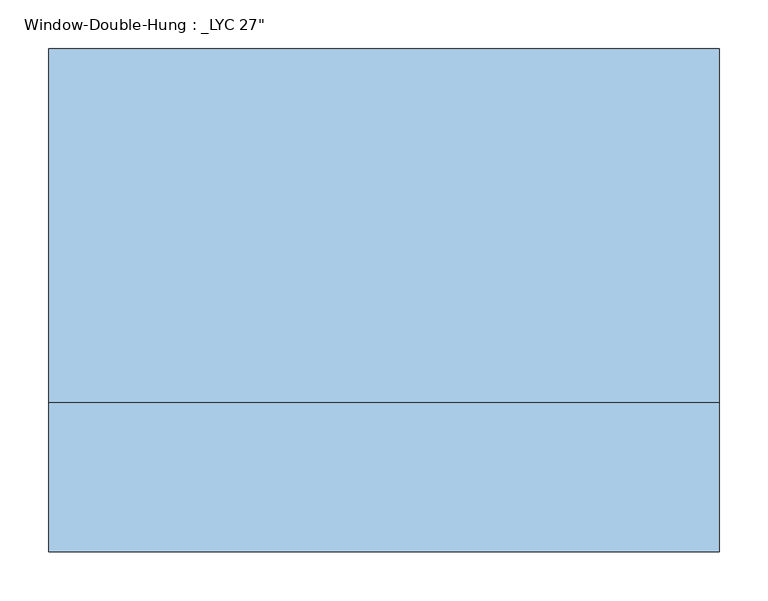
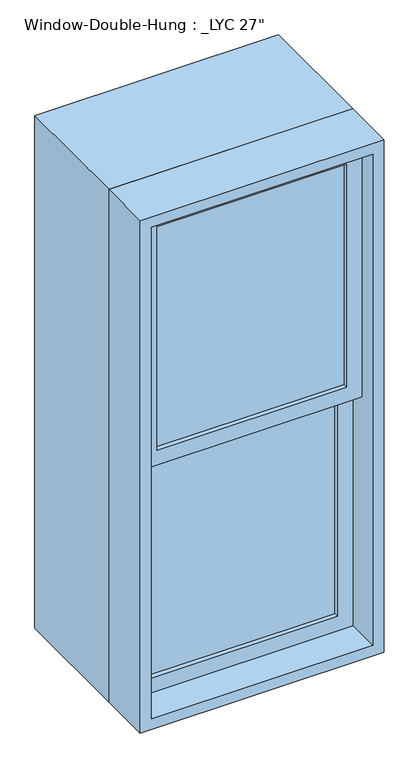
"""IFC4 building model written with IfcOpenShell, lengths in millimetres: window geometry."""

from ifc_helpers import new_model, si_unit, frame, origin, place, context, project, spatial, polyline, outline, extrude, source, transform, mapped, element, save


def window_2f9f7d73(model_context):
    return source(origin(), model_context, "Body", "SweptSolid", [
        extrude(outline(polyline([(266.7, -158.75), (-266.7, -158.75), (-266.7, -152.4), (266.7, -152.4), (266.7, -158.75)])), frame((0.0, 0.0, 990.6), z_axis=(0.0, 0.0, 1.0), x_axis=(1.0, 0.0, 0.0)), (0.0, 0.0, 1.0), 663.575),
        extrude(outline(polyline([(-266.7, -146.05), (-266.7, -139.7), (266.7, -139.7), (266.7, -146.05), (-266.7, -146.05)])), frame((0.0, 0.0, 990.6), z_axis=(0.0, 0.0, 1.0), x_axis=(1.0, 0.0, 0.0)), (0.0, 0.0, 1.0), 663.575),
        extrude(outline(polyline([(266.7, -203.2), (-266.7, -203.2), (-266.7, -196.85), (266.7, -196.85), (266.7, -203.2)])), frame((0.0, 0.0, 1698.625), z_axis=(0.0, 0.0, 1.0), x_axis=(1.0, 0.0, 0.0)), (0.0, 0.0, 1.0), 663.575),
        extrude(outline(polyline([(-266.7, -190.5), (-266.7, -184.15), (266.7, -184.15), (266.7, -190.5), (-266.7, -190.5)])), frame((0.0, 0.0, 1698.625), z_axis=(0.0, 0.0, 1.0), x_axis=(1.0, 0.0, 0.0)), (0.0, 0.0, 1.0), 663.575),
        extrude(outline(polyline([(1698.625, 311.15), (1698.625, -311.15), (946.15, -311.15), (946.15, 311.15), (1698.625, 311.15)]), holes=[polyline([(1654.175, -266.7), (1654.175, 266.7), (990.6, 266.7), (990.6, -266.7), (1654.175, -266.7)])]), frame((0.0, -171.45, 0.0), z_axis=(0.0, 1.0, 0.0), x_axis=(0.0, 0.0, 1.0)), (0.0, 0.0, 1.0), 44.45),
        extrude(outline(polyline([(2406.65, 311.15), (2406.65, -311.15), (1654.175, -311.15), (1654.175, 311.15), (2406.65, 311.15)]), holes=[polyline([(2362.2, -266.7), (2362.2, 266.7), (1698.625, 266.7), (1698.625, -266.7), (2362.2, -266.7)])]), frame((0.0, -215.9, 0.0), z_axis=(0.0, 1.0, 0.0), x_axis=(0.0, 0.0, 1.0)), (0.0, 0.0, 1.0), 44.45),
        extrude(outline(polyline([(2438.4, 342.9), (2438.4, -342.9), (914.4, -342.9), (914.4, 342.9), (2438.4, 342.9)]), holes=[polyline([(2406.65, -311.15), (2406.65, 311.15), (946.15, 311.15), (946.15, -311.15), (2406.65, -311.15)])]), frame((0.0, -266.7, 0.0), z_axis=(0.0, 1.0, 0.0), x_axis=(0.0, 0.0, 1.0)), (0.0, 0.0, 1.0), 152.4),
        extrude(outline(polyline([(2438.4, 342.9), (2438.4, -342.9), (914.4, -342.9), (914.4, 342.9), (2438.4, 342.9)]), holes=[polyline([(2419.35, 323.85), (933.45, 323.85), (933.45, -323.85), (2419.35, -323.85), (2419.35, 323.85)])]), frame((0.0, -114.3, 0.0), z_axis=(0.0, 1.0, 0.0), x_axis=(0.0, 0.0, 1.0)), (0.0, 0.0, 1.0), 361.95),
    ])


if __name__ == "__main__":
    model = new_model("IFC4")
    model_context = context("Model", 3, world=origin())
    ifc_project = project(units=[si_unit("LENGTHUNIT", "METRE", prefix="MILLI")], contexts=[model_context])
    site = spatial("IfcSite", under=ifc_project)
    building = spatial("IfcBuilding", under=site)
    placement = place(None, origin())
    window_shape = window_2f9f7d73(model_context)
    element("IfcWindow", 1, ObjectType="Window-Double-Hung : _LYC 27\"", at=placement, inside=building, context=model_context, shape_type="MappedRepresentation", body=[
        mapped(window_shape, transform((0.0, 0.0, 0.0), x_axis=(1.0, 0.0, 0.0), y_axis=(0.0, 1.0, 0.0), z_axis=(0.0, 0.0, 1.0))),
    ])
    save(model, "model.ifc")

# Revit data of these elements
# Type "Window-Double-Hung : _LYC 27\""
#   Type Mark = "24"
#   Fire Rating = "0.5h"
#   Assembly Code = "B2020100"
#   Wall Thickness [instance default] = 0' - 6"
#   Visual Light Transmittance = 0.9
#   Thermal Resistance (R) = 1.8146 (h·ft²·°F)/BTU
#   Solar Heat Gain Coefficient = 0.78
#   Rough Width = 2' - 3 1/2"
#   Rough Height = 5' - 0 1/2"
#   Muntin Width = 1' - 9"
#   Muntin Height = 2' - 2 1/8"
#   Interior Wall Closure [instance default] = 0' - 1 1/2"
#   Heat Transfer Coefficient (U) = 0.6496 BTU/(h·ft²·°F)
#   Frame Extension [instance default] = 0' - 2"
#   Exterior Wall Closure [instance default] = 0' - 0 1/2"
#   Extension Jamb [instance default] = 0' - 0 3/4"
#   Height = 5' - 0"
#   Width = 2' - 3"
#   Window Inset [instance default] = 0' - 0 3/4"
#   Top Muntin Visibility = yes
#   Interior Trim Visibility [instance default] = yes
#   Indicator Visibility [instance default] = yes
#   Exterior Trim Visibility [instance default] = yes
#   Extension Jamb Visibility [instance default] = yes
#   Define Thermal Properties by = 1
#   Bottom Muntin Visibility = yes
#   Muntin Pattern = Muntin Pattern_2x2 : Muntin Pattern_2x2
#   Interior Trim Material = Wood - Stained
#   Interior Trim = Trim-Window-Interior-Flat : Picture Frame
#   Interior Frame Material = Wood - Stained
#   Glass Panel Material = Glass
#   Exterior Trim Material = Clad - White
#   Exterior Trim = Trim-Window-Exterior-Flat : with Sill
#   Exterior Frame Material = Clad - White
#   Construction Type Id = ""
#   Wall Closure = (empty or 0)
#   Analytic Construction = (empty or 0)
# Element 1 (IfcWindow, "Window-Double-Hung : _LYC 27\"")
#   Wall Thickness = 1' - 7 1/2"
#   Extension Jamb = 1' - 2 1/4"
#   Materials on its faces: "Wood - Stained", "Glass", "Clad - White"
# Materials
#   "Wood - Stained": class "Wood", colour RGB 224 178 126, transparency 0, Cost = 0
#   "Glass": class "Unassigned", colour RGB 0 128 192, transparency 0.75
#   "Clad - White": class "Wood", colour RGB 242 242 238, transparency 0, Cost = 0
